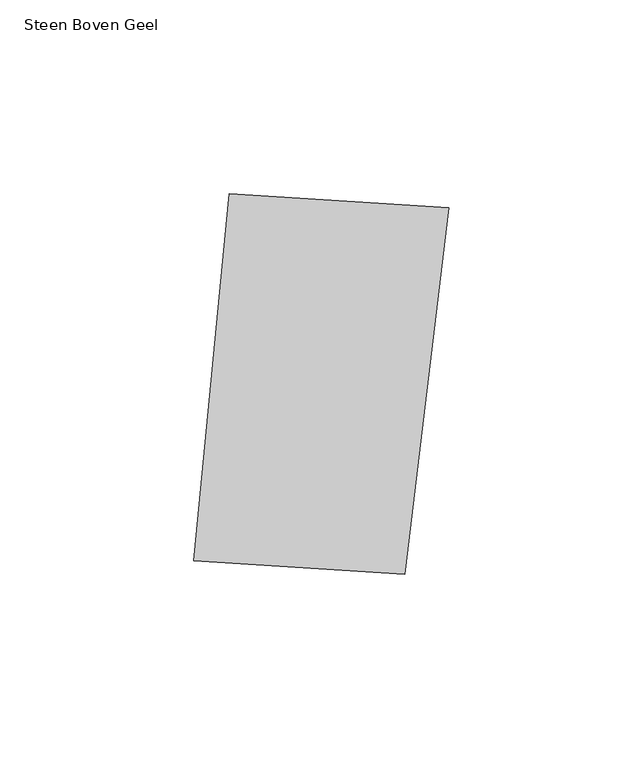
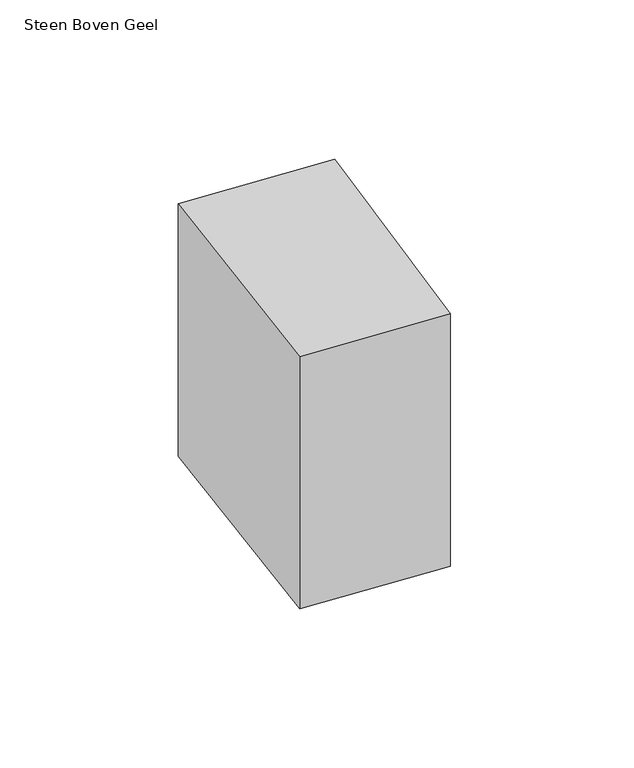
"""IFC4 building model written with IfcOpenShell, lengths in millimetres: proxy geometry, 00_GMA_steen_versie_4 : Steen Boven Geel."""

from ifc_helpers import new_model, si_unit, origin, origin_with_axes, place, context, project, spatial, polyline, outline, extrude, source, transform, mapped, element, save


def steen_boven_geel_41e19b64(model_context):
    return source(origin(), model_context, "Body", "SweptSolid", [
        extrude(outline(polyline([(106.4950074, 118.6367934), (95.2235394, 24.1529126), (40.7776205, 27.6045809), (49.9415995, 122.2177388), (106.4950074, 118.6367934)])), origin_with_axes(), (0.0, 0.0, 1.0), 100.0),
    ])


if __name__ == "__main__":
    model = new_model("IFC4")
    model_context = context("Model", 3, world=origin())
    ifc_project = project(units=[si_unit("LENGTHUNIT", "METRE", prefix="MILLI")], contexts=[model_context])
    site = spatial("IfcSite", under=ifc_project)
    building = spatial("IfcBuilding", under=site)
    placement = place(None, origin())
    steen_boven_geel_shape = steen_boven_geel_41e19b64(model_context)
    element("IfcBuildingElementProxy", 1, Name="00_GMA_steen_versie_4 : Steen Boven Geel", ObjectType="00_GMA_steen_versie_4 : Steen Boven Geel", at=placement, inside=building, context=model_context, shape_type="MappedRepresentation", body=[
        mapped(steen_boven_geel_shape, transform((0.0, 0.0, 0.0), x_axis=(1.0, 0.0, 0.0), y_axis=(0.0, 1.0, 0.0), z_axis=(0.0, 0.0, 1.0))),
    ])
    save(model, "model.ifc")

# Revit data of these elements
# Type "00_GMA_steen_versie_4 : Steen Boven Geel"
#   StootVoegHalfBoven [instance default] = 5 mm
#   StootVoegHalf [instance default] = 5 mm
#   StootVoegBreedteOnder = 10 mm
#   StootVoegBreedteBoven = 10 mm
#   Steendikte = 100 mm
#   LintVoegOnderHalf = 5 mm
#   LintVoegOnder = 10 mm
#   LintVoegBovenHalf = 0 mm
#   LintVoegBoven = 0 mm
#   materiaal = 21_steen_geel
#   MateriaalVoeg = none
#   Default Elevation = 0
# Element 1 (IfcBuildingElementProxy, "00_GMA_steen_versie_4 : Steen Boven Geel")
#   Materials on its faces: "21_steen_geel"
# Materials
#   "21_steen_geel": class "Unassigned", colour RGB 202 202 0, transparency 0, Cost = 0
